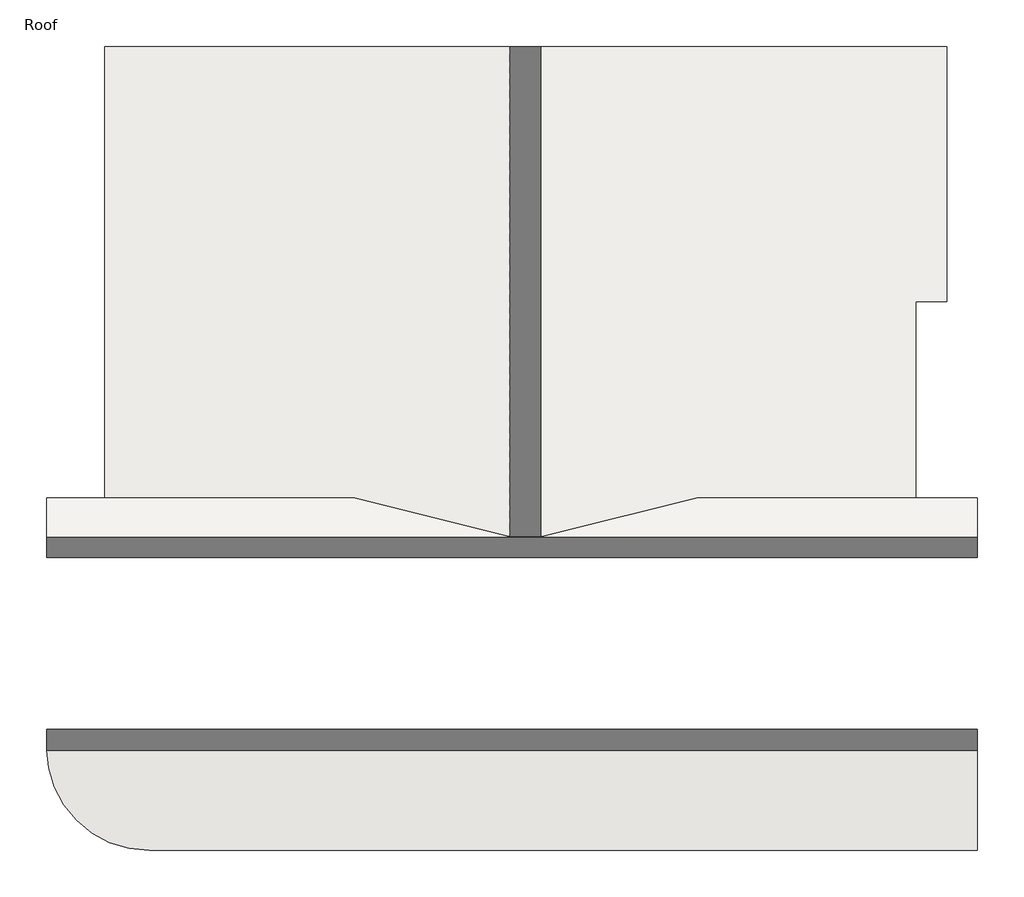
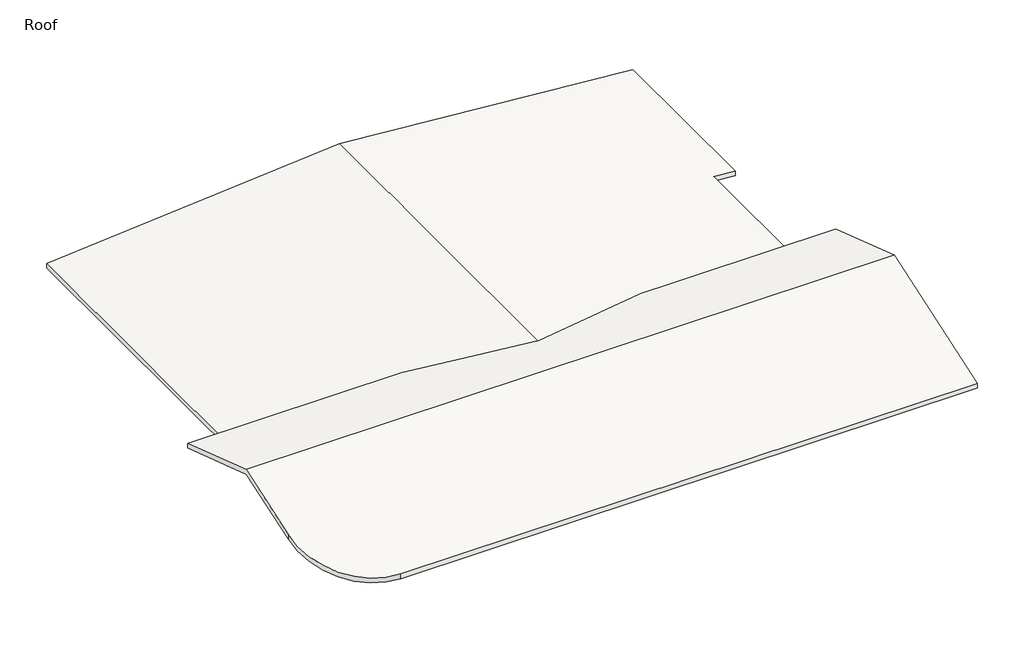
# One storey: 3 walls, 2 roofs.
"""IFC4 building model written with IfcOpenShell, lengths in millimetres."""

import ifcopenshell
import ifcopenshell.guid

model = None  # the IFC model being written
_history = None  # IfcOwnerHistory: only IFC2X3 demands one
_inside = {}  # id of a spatial element -> (the spatial element, [elements in it])
_under = {}  # id of a project, library or spatial element -> (it, [spatial elements below it])
_declared = {}  # id of a project -> (the project, [libraries it declares])
_typed = {}  # id of a type object -> (the type object, [elements of that type])
_made_of = {}  # id of a material, layer set ... -> (it, [elements and type objects made of it])


def new_model(schema):
    """Start an empty IFC model of exactly this schema.

    Asked for "IFC4X3", IfcOpenShell would pick the latest addendum, in which some entities
    have other attributes; the version numbers below select the first issue.
    IFC2X3 requires an IfcOwnerHistory on every rooted entity: one is made here for all.
    """
    global model, _history
    if schema == "IFC4X3":
        model = ifcopenshell.file(schema_version=(4, 3, 0, 0))
    else:
        model = ifcopenshell.file(schema=schema)
    _inside.clear()
    _under.clear()
    _declared.clear()
    _typed.clear()
    _made_of.clear()
    _history = None
    if model.schema == "IFC2X3":
        org = make("IfcOrganization", Name="unknown")
        user = make(
            "IfcPersonAndOrganization",
            ThePerson=make("IfcPerson", FamilyName="unknown"),
            TheOrganization=org,
        )
        app = make(
            "IfcApplication",
            ApplicationDeveloper=org,
            Version="unknown",
            ApplicationFullName="unknown",
            ApplicationIdentifier="unknown",
        )
        _history = make(
            "IfcOwnerHistory",
            OwningUser=user,
            OwningApplication=app,
            ChangeAction="ADDED",
            CreationDate=0,
        )
    return model


def make(cls, **values):
    """One entity of the class cls with the attributes given. An attribute that is None is left unset."""
    return model.create_entity(
        cls, **{name: value for name, value in values.items() if value is not None}
    )


def rooted(cls, **values):
    """An entity with a GlobalId (a new one), such as an element, a storey or a relation."""
    return make(cls, GlobalId=ifcopenshell.guid.new(), OwnerHistory=_history, **values)


def si_unit(unit_type, name, prefix=None):
    """IfcSIUnit, for example si_unit("LENGTHUNIT", "METRE", prefix="MILLI")."""
    return make("IfcSIUnit", UnitType=unit_type, Prefix=prefix, Name=name)


def assignment(units):
    """IfcUnitAssignment: the units of a project."""
    return None if units is None else make("IfcUnitAssignment", Units=units)


def point(xyz):
    """IfcCartesianPoint."""
    return None if xyz is None else make("IfcCartesianPoint", Coordinates=xyz)


def direction(xyz):
    """IfcDirection."""
    return None if xyz is None else make("IfcDirection", DirectionRatios=xyz)


def frame(location, z_axis=None, x_axis=None):
    """IfcAxis2Placement3D, a coordinate frame: its origin and axes. An axis left out is left unset."""
    return make(
        "IfcAxis2Placement3D",
        Location=point(location),
        Axis=direction(z_axis),
        RefDirection=direction(x_axis),
    )


def origin():
    """The frame at (0, 0, 0) with its axes left unset."""
    return frame((0.0, 0.0, 0.0))


def place(relative_to, where):
    """IfcLocalPlacement: puts the frame where relative to a parent placement (None: the world)."""
    return make(
        "IfcLocalPlacement", PlacementRelTo=relative_to, RelativePlacement=where
    )


def context(
    kind, dimensions, precision=None, world=None, true_north=None, identifier=None
):
    """IfcGeometricRepresentationContext, for example the 3D "Model" context."""
    return make(
        "IfcGeometricRepresentationContext",
        ContextIdentifier=identifier,
        ContextType=kind,
        CoordinateSpaceDimension=dimensions,
        Precision=precision,
        WorldCoordinateSystem=world,
        TrueNorth=true_north,
    )


def project(units=None, contexts=None):
    """IfcProject with its units and contexts."""
    return rooted(
        "IfcProject",
        Name="project",
        RepresentationContexts=contexts,
        UnitsInContext=assignment(units),
    )


def spatial(cls, under=None, at=None, **own):
    """A site, building, storey or space (cls), placed at a placement, below another one or the project."""
    s = rooted(cls, ObjectPlacement=at, **own)
    if under is not None:
        _under.setdefault(under.id(), (under, []))[1].append(s)
    return s


def polyline(points):
    """IfcPolyline through the points."""
    return make("IfcPolyline", Points=[point(p) for p in points])


def ellipse_curve(where, semi_axis1, semi_axis2):
    """IfcEllipse in the frame where."""
    return make(
        "IfcEllipse", Position=where, SemiAxis1=semi_axis1, SemiAxis2=semi_axis2
    )


def outline(outer, holes=None, kind="AREA"):
    """IfcArbitraryClosedProfileDef: a profile drawn as a closed curve; with holes, ...WithVoids."""
    if holes is None:
        return make("IfcArbitraryClosedProfileDef", ProfileType=kind, OuterCurve=outer)
    return make(
        "IfcArbitraryProfileDefWithVoids",
        ProfileType=kind,
        OuterCurve=outer,
        InnerCurves=holes,
    )


def extrude(swept, where, along, depth):
    """IfcExtrudedAreaSolid: the profile swept, set in the frame where, extruded along a direction by depth."""
    return make(
        "IfcExtrudedAreaSolid",
        SweptArea=swept,
        Position=where,
        ExtrudedDirection=direction(along),
        Depth=depth,
    )


def faces_of(points, faces, orient=None, outer=None):
    """IfcFace entities. A face is a list of loops; a loop is a list of indices into points, from 0.

    orient and outer hold one flag for each loop. By default every Orientation is true, the
    first loop of a face is its IfcFaceOuterBound and the others are IfcFaceBound.
    """
    made = []
    for i, loops in enumerate(faces):
        bounds = []
        for j, loop in enumerate(loops):
            is_outer = j == 0 if outer is None else outer[i][j]
            bounds.append(
                make(
                    "IfcFaceOuterBound" if is_outer else "IfcFaceBound",
                    Bound=make("IfcPolyLoop", Polygon=[points[k] for k in loop]),
                    Orientation=True if orient is None else orient[i][j],
                )
            )
        made.append(make("IfcFace", Bounds=bounds))
    return made


def faceted_brep(points, faces, orient=None, outer=None, voids=None):
    """IfcFacetedBrep: a solid bounded by flat faces; with voids (closed shells), ...WithVoids."""
    shared = [point(p) for p in points]
    hull = make("IfcClosedShell", CfsFaces=faces_of(shared, faces, orient, outer))
    if voids is None:
        return make("IfcFacetedBrep", Outer=hull)
    return make(
        "IfcFacetedBrepWithVoids",
        Outer=hull,
        Voids=[
            make(cls, CfsFaces=faces_of(shared, fs, o, b)) for cls, fs, o, b in voids
        ],
    )


def shape(context_of_items, identifier, shape_type, items):
    """IfcShapeRepresentation: the items that make up one representation, for example the "Body"."""
    return make(
        "IfcShapeRepresentation",
        ContextOfItems=context_of_items,
        RepresentationIdentifier=identifier,
        RepresentationType=shape_type,
        Items=items,
    )


def made_of(thing, what):
    """Note that an element or type object is made of a material, layer set ...; save() writes the relation."""
    if what is not None:
        _made_of.setdefault(what.id(), (what, []))[1].append(thing)
    return thing


def element(
    cls,
    number,
    at=None,
    inside=None,
    cuts=None,
    type_object=None,
    material=None,
    context=None,
    identifier="Body",
    shape_type=None,
    held_by="IfcProductDefinitionShape",
    body=None,
    shapes=None,
    **own,
):
    """One element of the class cls, such as IfcWall. Its Tag is "e" and its number.

    at: its placement. inside: the storey or other place that contains it. cuts: it is an
    opening in that element (IfcRelVoidsElement). A single representation is given by context,
    identifier, shape_type and body (its items); several are given by shapes. held_by: the class
    of the entity that holds the representations. save() writes the other relations.
    """
    e = rooted(cls, Tag="e%d" % number, ObjectPlacement=at, **own)
    if body is not None:
        shapes = [shape(context, identifier, shape_type, body)]
    if shapes is not None:
        e.Representation = make(held_by, Representations=shapes)
    if inside is not None:
        _inside.setdefault(inside.id(), (inside, []))[1].append(e)
    if cuts is not None:
        rooted(
            "IfcRelVoidsElement", RelatingBuildingElement=cuts, RelatedOpeningElement=e
        )
    if type_object is not None:
        _typed.setdefault(type_object.id(), (type_object, []))[1].append(e)
    return made_of(e, material)


def aggregate(whole, parts):
    """IfcRelAggregates: a whole, such as a stair, and the parts it consists of."""
    return rooted("IfcRelAggregates", RelatingObject=whole, RelatedObjects=parts)


def save(model, path):
    """Write the relations noted so far, then the file.

    IfcRelAggregates (storeys below a building ...), IfcRelContainedInSpatialStructure (elements
    in a storey), IfcRelDefinesByType, IfcRelAssociatesMaterial and IfcRelDeclares: one each for
    every whole, place, type object, material and project.
    """
    for whole, parts in _under.values():
        aggregate(whole, parts)
    for where, things in _inside.values():
        rooted(
            "IfcRelContainedInSpatialStructure",
            RelatedElements=things,
            RelatingStructure=where,
        )
    for kind, things in _typed.values():
        rooted("IfcRelDefinesByType", RelatedObjects=things, RelatingType=kind)
    for what, things in _made_of.values():
        rooted("IfcRelAssociatesMaterial", RelatedObjects=things, RelatingMaterial=what)
    for by, libraries in _declared.values():
        rooted("IfcRelDeclares", RelatingContext=by, RelatedDefinitions=libraries)
    model.write(path)


def plane_surface(at):
    """IfcPlane: the flat surface through the origin of the frame at, square to its z axis."""
    return make("IfcPlane", Position=at)


def cylinder_surface(at, radius):
    """IfcCylindricalSurface: all points at the distance radius from the z axis of the frame at."""
    return make("IfcCylindricalSurface", Position=at, Radius=radius)


def advanced_brep(points, edges, surfaces, faces):
    """IfcAdvancedBrep: a solid bounded by faces that lie on surfaces and meet in shared edges.

    An edge is (start, end): straight between two places in points (the first is 0);
    or (start, end, curve); or (start, end, curve, False) where it runs against its curve.
    A face is (place in surfaces, loops), or (place, loops, False) where it looks against
    its surface's normal. A loop lists edges by number (the first is 1), with a minus sign
    where the edge is run from its end to its start. The first loop is the outer one.
    """
    corners = [point(p) for p in points]
    vertices = [make("IfcVertexPoint", VertexGeometry=c) for c in corners]
    made = []
    for start, end, *more in edges:
        made.append(
            make(
                "IfcEdgeCurve",
                EdgeStart=vertices[start],
                EdgeEnd=vertices[end],
                EdgeGeometry=more[0] if more else make("IfcPolyline", Points=[corners[start], corners[end]]),
                SameSense=more[1] if len(more) > 1 else True,
            )
        )
    hull = []
    for where, loops, *sense in faces:
        bounds = []
        for j, loop in enumerate(loops):
            ring = [make("IfcOrientedEdge", EdgeElement=made[abs(k) - 1], Orientation=k > 0) for k in loop]
            bounds.append(
                make(
                    "IfcFaceOuterBound" if j == 0 else "IfcFaceBound",
                    Bound=make("IfcEdgeLoop", EdgeList=ring),
                    Orientation=True,
                )
            )
        hull.append(make("IfcAdvancedFace", Bounds=bounds, FaceSurface=surfaces[where], SameSense=sense[0] if sense else True))
    return make("IfcAdvancedBrep", Outer=make("IfcClosedShell", CfsFaces=hull))


model = new_model("IFC4")

# Units and contexts
model_context = context("Model", 3, world=origin())
ifc_project = project(units=[si_unit("LENGTHUNIT", "METRE", prefix="MILLI")], contexts=[model_context])

# Site, building, storey
site = spatial("IfcSite", under=ifc_project)
building = spatial("IfcBuilding", under=site)
storey = spatial("IfcBuildingStorey", under=building, Name="Roof", Elevation=9144.0)

# Roofs
placement = place(None, origin())
element("IfcRoof", 1, ObjectType="Insulation on Metal Deck - EPDM", at=placement, inside=storey, context=model_context, shape_type="AdvancedBrep", body=[
    advanced_brep(
    [(11609.8492079, -14879.2601743, 11192.9333333), (11609.8492079, -21026.0601743, 9144.0), (-12977.3507921, -21026.0601743, 9144.0), (-16025.3507921, -17978.0601743, 10160.0), (-16025.3507921, -14879.2601743, 11192.9333333), (-16025.3507921, -10561.2601743, 9753.6), (11609.8492079, -10561.2601743, 9753.6), (11609.8492079, -21026.0601743, 9351.4981191), (11609.8492079, -14879.2601743, 11400.4314525), (-16025.3507921, -14879.2601743, 11400.4314525), (-16025.3507921, -17978.0601743, 10367.4981191), (-12977.3507921, -21026.0601743, 9351.4981191), (11609.8492079, -10561.2601743, 9961.0981191), (-16025.3507921, -10561.2601743, 9961.0981191)],
    [
        (0, 1),
        (1, 2),
        (2, 3, ellipse_curve(frame((-12977.3507921, -17978.0601743, 10160.0), z_axis=(0.0, 0.316227766016838, -0.9486832980505139), x_axis=(0.0, 0.9486832980505139, 0.31622776601683744)), 3212.8741027, 3048.0)),
        (3, 4),
        (4, 0),
        (5, 6),
        (6, 0),
        (4, 5),
        (7, 8),
        (8, 9),
        (9, 10),
        (10, 11, ellipse_curve(frame((-12977.3507921, -17978.0601743, 10367.4981191), z_axis=(0.0, -0.316227766016838, 0.9486832980505139), x_axis=(0.0, 0.9486832980505139, 0.31622776601683744)), 3212.8741027, 3048.0)),
        (11, 7),
        (12, 13),
        (13, 9),
        (8, 12),
        (5, 13),
        (12, 6),
        (1, 7),
        (11, 2),
        (3, 10),
    ],
    [
        plane_surface(frame((-12977.3507921, -21026.0601743, 9144.0), z_axis=(0.0, 0.316227766016838, -0.9486832980505139), x_axis=(1.0, 0.0, 0.0))),
        plane_surface(frame((11609.8492079, -10561.2601743, 9753.6), z_axis=(0.0, -0.316227766016838, -0.9486832980505139), x_axis=(-1.0, 0.0, 0.0))),
        plane_surface(frame((-12977.3507921, -21026.0601743, 9351.4981191), z_axis=(0.0, -0.316227766016838, 0.9486832980505139), x_axis=(1.0, 0.0, 0.0))),
        plane_surface(frame((11609.8492079, -10561.2601743, 9961.0981191), z_axis=(0.0, 0.316227766016838, 0.9486832980505139), x_axis=(-1.0, 0.0, 0.0))),
        plane_surface(frame((-2207.7507921, -10561.2601743, 9753.6), z_axis=(0.0, 1.0, 0.0), x_axis=(-1.0, 0.0, 0.0))),
        plane_surface(frame((-683.7507921, -21026.0601743, 9144.0), z_axis=(0.0, -1.0, 0.0), x_axis=(1.0, 0.0, 0.0))),
        plane_surface(frame((11609.8492079, -21026.0601743, 9144.0), z_axis=(1.0, 0.0, 0.0), x_axis=(0.0, 1.0, 0.0))),
        plane_surface(frame((-16025.3507921, -10561.2601743, 9144.0), z_axis=(-1.0, 0.0, 0.0), x_axis=(0.0, -1.0, 0.0))),
        cylinder_surface(frame((-12977.3507921, -17978.0601743, 9144.0), z_axis=(0.0, 0.0, 1.0), x_axis=(0.0, -1.0, 0.0)), 3048.0),
    ],
    [
        (0, [[1, 2, 3, 4, 5]]),
        (1, [[6, 7, -5, 8]]),
        (2, [[9, 10, 11, 12, 13]]),
        (3, [[14, 15, -10, 16]]),
        (4, [[17, -14, 18, -6]]),
        (5, [[19, -13, 20, -2]]),
        (6, [[-16, -9, -19, -1, -7, -18]]),
        (7, [[-11, -15, -17, -8, -4, 21]]),
        (8, [[-12, -21, -3, -20]]),
    ],
),
])
element("IfcRoof", 2, ObjectType="Insulation on Metal Deck - EPDM", at=placement, inside=storey, context=model_context, shape_type="Brep", body=[
    faceted_brep([(-1801.3507921, 2849.9398257, 10185.4), (10695.4492079, 2849.9398257, 9144.0), (10695.4492079, -4719.2601743, 9144.0), (9781.0492079, -4719.2601743, 9220.2), (9781.0492079, -11170.8601743, 9220.2), (3380.2492079, -11170.8601743, 9753.6), (3380.2492079, -10561.2601743, 9753.6), (890.2717782, -10561.2601743, 9961.0981191), (-1801.3507921, -11234.1658169, 10185.4), (-14298.1507921, -11780.4601743, 9144.0), (-14298.1507921, 2849.9398257, 9144.0), (-1953.7507921, -11196.0658169, 10172.7), (-4492.9733625, -10561.2601743, 9961.0981191), (-6982.9507921, -10561.2601743, 9753.6), (-6982.9507921, -11780.4601743, 9753.6), (10695.4492079, 2849.9398257, 9341.5323244), (-1801.3507921, 2849.9398257, 10382.9323244), (-1801.3507921, -11826.7627901, 10382.9323244), (3260.6596711, -10561.2601743, 9961.0981191), (5750.6371007, -10561.2601743, 9753.6), (5750.6371007, -11170.8601743, 9753.6), (9781.0492079, -11170.8601743, 9417.7323244), (9781.0492079, -4719.2601743, 9417.7323244), (10695.4492079, -4719.2601743, 9341.5323244), (-14298.1507921, 2849.9398257, 9341.5323244), (-14298.1507921, -11780.4601743, 9341.5323244), (-9353.338685, -11780.4601743, 9753.6), (-9353.338685, -10561.2601743, 9753.6), (-6863.3612554, -10561.2601743, 9961.0981191), (-1953.7507921, -11788.6627901, 10370.2323244)], [[[0, 1, 2, 3, 4, 5, 6, 7, 8]], [[9, 10, 0, 8, 11, 12, 13, 14]], [[15, 16, 17, 18, 19, 20, 21, 22, 23]], [[24, 25, 26, 27, 28, 29, 17, 16]], [[9, 25, 24, 10]], [[1, 15, 23, 2]], [[24, 16, 15, 1, 0, 10]], [[23, 22, 3, 2]], [[22, 21, 4, 3]], [[26, 25, 9, 14]], [[26, 14, 13, 27]], [[29, 28, 12, 11]], [[28, 27, 13, 12]], [[21, 20, 5, 4]], [[5, 20, 19, 6]], [[19, 18, 7, 6]], [[18, 17, 29, 11, 8, 7]]]),
])

# Walls
element("IfcWall", 3, ObjectType="Generic - 12\"", at=placement, inside=storey, context=model_context, shape_type="Brep", body=[
    faceted_brep([(9781.0492079, -11170.8601743, 9144.0), (-1953.7507921, -11170.8601743, 9144.0), (-1953.7507921, -11170.8601743, 9956.8), (9781.0492079, -11170.8601743, 9956.8), (9781.0492079, -11475.6601743, 9144.0), (9781.0492079, -11475.6601743, 10058.4), (-1648.9507921, -11475.6601743, 10058.4), (-1953.7507921, -11475.6601743, 10058.4), (-1953.7507921, -11475.6601743, 9144.0), (-1648.9507921, -11475.6601743, 9144.0)], [[[0, 1, 2, 3]], [[4, 5, 6, 7, 8, 9]], [[1, 0, 4, 9, 8]], [[2, 1, 8, 7]], [[0, 3, 5, 4]], [[3, 2, 7, 6, 5]]]),
])
element("IfcWall", 4, ObjectType="Generic - 12\"", at=placement, inside=storey, context=model_context, shape_type="Brep", body=[
    faceted_brep([(-1953.7507921, -11475.6601743, 9144.0), (-1953.7507921, -11780.4601743, 9144.0), (-1953.7507921, -12085.2601743, 9144.0), (-1953.7507921, -12085.2601743, 10261.6), (-1953.7507921, -11780.4601743, 10160.0), (-1953.7507921, -11475.6601743, 10058.4), (-1648.9507921, -11475.6601743, 9144.0), (-1648.9507921, -11475.6601743, 10058.4), (-1648.9507921, -12085.2601743, 10261.6), (-1648.9507921, -12085.2601743, 9144.0)], [[[0, 1, 2, 3, 4, 5]], [[6, 7, 8, 9]], [[2, 1, 0, 6, 9]], [[0, 5, 7, 6]], [[3, 2, 9, 8]], [[5, 4, 3, 8, 7]]]),
])
element("IfcWall", 5, ObjectType="Generic - 12\"", at=placement, inside=storey, context=model_context, shape_type="SweptSolid", body=[
    extrude(outline(polyline([(-12085.2601743, 9144.0), (-12085.2601743, 10261.6), (-11780.4601743, 10160.0), (-11780.4601743, 9144.0), (-12085.2601743, 9144.0)])), frame((-14298.1507921, 0.0, 0.0), z_axis=(1.0, 0.0, 0.0), x_axis=(0.0, 1.0, 0.0)), (0.0, 0.0, 1.0), 12344.4),
])

save(model, "model.ifc")

# Revit data of these elements
# Project information
#   Project Issue Date = "Issue Date"
#   Project Status = "Project Status"
#   Client Name = "Owner"
#   Project Address = "Enter address here"
#   Project Name = "Project Name"
#   Project Number = "Project Number"
# Grids (mm)
#   "1": line (14427.416, 17480.34) -> (-18533.688, 17480.34)
#   "2": line (14427.416, 10165.14) -> (-18533.688, 10165.14)
#   "3": line (14427.416, 2849.94) -> (-18533.688, 2849.94)
#   "4": line (14427.416, -4465.26) -> (-18533.688, -4465.26)
#   "5": line (14427.416, -11780.46) -> (-18533.688, -11780.46)
#   "6": line (14427.416, -19095.66) -> (-18533.688, -19095.66)
#   "A": line (-13993.351, 21295.126) -> (-13993.351, -21386.076)
#   "B": line (-5458.951, 21295.126) -> (-5458.951, -21386.076)
#   "C": line (3075.449, 21295.126) -> (3075.449, -21386.076)
#   "D": line (10390.649, 21295.126) -> (10390.649, -21386.076)
# Type "Insulation on Metal Deck - EPDM"
#   Assembly Code = "B1020"
#   Layers, outside or top first: 0' - 0 1/4" "Roofing, EPDM Membrane" (function 4); 0' - 3" "Rigid insulation" (function 3); 0' - 3" "Concrete, Cast-in-Place gray" (function 1); 0' - 1 1/2" "Metal Deck" (function 1)
# Type "Generic - 12\""
#   Assembly Code = "B2010"
#   Layers, outside or top first: 1' - 0" no material (function 1)
# Element 1 (IfcRoof, "Insulation on Metal Deck - EPDM")
#   built-in parameter 1001705 = 37.403 (stored number, unit not read)
#   built-in parameter 1001710 = 33615
#   Phase Created = New Construction
#   Materials on its faces: "Metal Deck", "Roofing, EPDM Membrane"
# Element 2 (IfcRoof, "Insulation on Metal Deck - EPDM")
#   built-in parameter 1001705 = 34.0647 (stored number, unit not read)
#   built-in parameter 1001710 = 33615
#   Phase Created = New Construction
#   Materials on its faces: "Metal Deck", "Roofing, EPDM Membrane"
# Elements 3, 4, 5 (IfcWall, "Generic - 12\"")
#   Top Offset = 0' - 0"
#   Base Offset = 0' - 0"
#   wall height = 3' - 0"
#   Phase Created = New Construction
#   Base Constraint = Roof
#   Top Constraint = Parapet
#   Materials on its faces: "Default Wall"
# Materials
#   "Roofing, EPDM Membrane": class "Generic", colour RGB 127 127 127, transparency 0, Description = "EPDM roof membrane", Cost = 0
#   "Rigid insulation": class "Generic", colour RGB 127 127 127, transparency 0, Description = "Rigid foam insulation board", Cost = 0
#   "Concrete, Cast-in-Place gray": class "Concrete", colour RGB 192 192 192, transparency 0, Description = "Cast-in-place concrete", Cost = 0
#   "Metal Deck": class "Metal", colour RGB 199 199 199, transparency 0, Description = "Steel, mill finish", Cost = 0
#   "Default Wall": class "Miscellaneous", colour RGB 127 127 127, transparency 0
